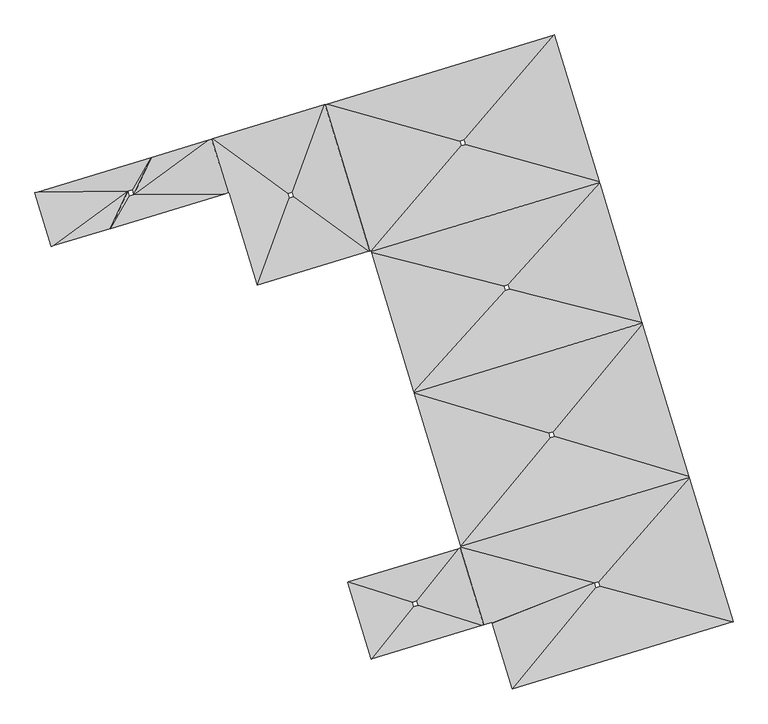
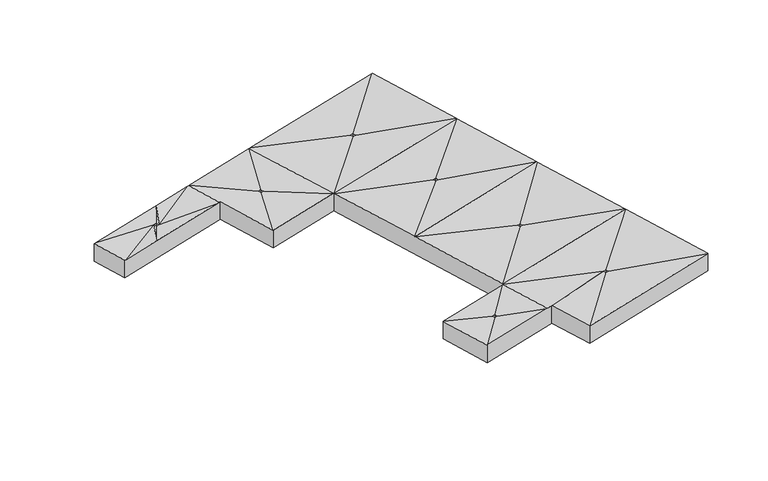
"""IFC4 building model written with IfcOpenShell, lengths in millimetres: proxy geometry, layer-410_topoId-1346273_creation_time-2021_Oct_27_15_18_18_ : layer-410_topoId-1346273_creation_time-2021_Oct_27_15_18_18_."""

from ifc_helpers import new_model, si_unit, origin, place, context, project, spatial, faceted_brep, source, transform, mapped, element, save


def generic_models_39dac30f(model_context):
    return source(origin(), model_context, "Body", "Brep", [
        faceted_brep([(28125.7662588, -17147.5862588, 474910.0155273), (10320.9487086, -22562.4314291, 474910.0155273), (8691.5481583, -17204.7223877, 474910.0155273), (-1028.2339046, -20160.7291608, 474910.0155273), (-2912.6258867, -13964.5670218, 474910.0155273), (6232.0389055, -11183.4693329, 474910.0155273), (-1053.4223403, 12772.2083054, 474910.0155273), (-10198.0872101, 9991.1094522, 474910.0155273), (-12471.5344882, 17466.5380451, 474910.0155273), (-26809.1523566, 13106.1448971, 474910.0155273), (-28125.7662527, 17435.3652172, 474910.0155273), (13736.4526166, 30166.6114523, 474910.0155273), (-20144.7843384, 17288.7016937, 474910.0155273), (-20261.1702576, 17671.3946136, 474910.0155273), (-20643.8631775, 17555.0086945, 474910.0155273), (-20527.4772583, 17172.3157745, 474910.0155273), (13370.0862305, -2328.9415649, 474910.0155273), (13752.7791504, -2212.5552097, 474910.0155273), (13636.3943939, -1829.8628712, 474910.0155273), (13253.7003113, -1946.247337, 474910.0155273), (10139.1450714, 9669.6086151, 474910.0155273), (10022.7579895, 10052.3026978, 474910.0155273), (9640.0656509, 9935.9167786, 474910.0155273), (9756.449826, 9553.2232773, 474910.0155273), (17312.0572449, -13915.987793, 474910.0155273), (16929.3631622, -14032.3713867, 474910.0155273), (17045.7490814, -14415.0654694, 474910.0155273), (17428.4420013, -14298.6795502, 474910.0155273), (2373.0752083, -15950.7356873, 474910.0155273), (2755.7692909, -15834.3486053, 474910.0155273), (2639.3830811, -15451.6545227, 474910.0155273), (2256.6897251, -15568.0416046, 474910.0155273), (6591.0546661, 21336.2557983, 474910.0155273), (6474.6681656, 21718.9487183, 474910.0155273), (6091.975827, 21602.5627991, 474910.0155273), (6208.3605835, 21219.8698792, 474910.0155273), (-7383.3045639, 17504.4268982, 474910.0155273), (-7765.9980652, 17388.040979, 474910.0155273), (-7649.612146, 17005.3468964, 474910.0155273), (-7266.9192261, 17121.7328156, 474910.0155273), (13736.4526166, 30166.6114523, 477196.9563735), (17337.0312354, 18327.3748578, 477196.9563736), (17355.6091377, 18266.2879591, 477200.0071289), (17373.1332797, 18208.6659809, 477196.9563739), (20786.012385, 6986.6132293, 477196.9563604), (20803.5365983, 6928.9910163, 477200.0071289), (20822.8041265, 6865.6365256, 477196.9563601), (24563.609524, -5434.6865183, 477196.956334), (24582.8772052, -5498.0415121, 477200.0071289), (24601.0541471, -5557.8099932, 477196.9563339), (28125.7662588, -17147.5862588, 477196.9563725), (10022.7579907, 10052.3026981, 476910.0154846), (10139.1450714, 9669.6086151, 476910.0155273), (9756.4498265, 9553.2232758, 476910.0154978), (2406.0771892, 1396.8605102, 477196.9570659), (2423.6012978, 1339.238641, 477200.0078163), (6591.0546661, 21336.2557983, 476910.0155273), (6208.3605834, 21219.8698796, 476910.0155364), (-1042.9065397, 12737.6241389, 477196.956431), (-1024.3258936, 12676.5348712, 477200.0073352), (-28125.7662527, 17435.3652172, 477197.264433), (-27898.7824792, 17504.3961093, 477190.7574194), (-18764.6808399, 20282.2827155, 477190.7574657), (-18748.8130647, 20287.1084643, 477192.2013141), (-14156.112444, 21683.8524513, 477192.2012927), (-13883.8217202, 21766.6622102, 477200.0071289), (-13811.6386368, 21788.6147162, 477196.711422), (-4811.3393377, 24525.8090088, 477196.7114045), (-4739.1558066, 24547.7616509, 477200.0071289), (-4589.3130727, 24593.3322105, 477195.2290651), (13682.2837137, 30150.1374655, 477195.2290779), (-20261.1702576, 17671.3946136, 476999.9821289), (-20144.7843384, 17288.7016937, 476999.9821289), (8020.7580555, -17408.7249131, 477200.0072194), (8691.5481608, -17204.722387, 477178.6175937), (8704.8017052, -17248.3019934, 477178.6175954), (16929.3631622, -14032.3713867, 476910.0155273), (6221.1191764, -11147.5636584, 477196.9562258), (6232.0389012, -11183.4693342, 477196.9562273), (6136.3656478, -11212.5657166, 477200.0069803), (2442.8686671, 1275.8846717, 477196.9562276), (13253.700312, -1946.2473395, 476910.0155846), (13636.3943939, -1829.8628712, 476910.0155273), (6474.6681656, 21718.9487183, 476910.0155273), (6202.9419645, -11087.794273, 477200.0067682), (17312.0572437, -13915.987789, 476910.0154428), (6183.6750397, -11024.4417655, 477196.9563724), (-1006.8017387, 12618.9128494, 477196.9563721), (-1053.4223403, 12772.2083054, 477196.956372), (9640.0656498, 9935.9167782, 476910.0154888), (13370.0862303, -2328.941565, 476910.015521), (13752.7791512, -2212.5552123, 476910.0154702), (28068.2902611, -17165.0660015, 477195.1236232), (10368.7396641, -22547.8971255, 477195.1236229), (10320.9487086, -22562.4314291, 477196.7504201), (17428.4420013, -14298.6795502, 476910.0155273), (17045.7490817, -14415.0654704, 476910.0155049), (7881.1577971, -17451.1805265, 477195.2267761), (-984.3046844, -20147.3692859, 477195.2266954), (-1028.2339046, -20160.7291608, 477196.7309708), (2755.7692909, -15834.3486053, 477049.9883789), (2373.0752065, -15950.7356815, 477049.9885037), (6091.9758266, 21602.5628004, 476910.0154974), (-12889.8650569, 17339.3142788, 477190.7574189), (-12567.2078521, 17437.4416161, 477200.0071289), (-2912.6258867, -13964.5670218, 477196.730971), (2256.6897251, -15568.0416046, 477049.9883789), (-2868.6966966, -13951.2070954, 477195.2267039), (-7383.3045648, 17504.4268979, 476999.9821493), (-7266.9192261, 17121.7328156, 476999.9821289), (-1221.2774175, 12721.1616295, 477196.7115505), (-1149.0957229, 12743.1118717, 477200.0071646), (-12471.5344882, 17466.5380451, 477195.6389198), (-22023.9665536, 14561.4278862, 477190.7574501), (-22039.8343554, 14556.6021296, 477192.201301), (-26632.5344618, 13159.8583846, 477192.2012731), (-26809.1523566, 13106.1448971, 477197.2644337), (-20527.4772591, 17172.3157772, 476999.982159), (8718.2324863, -17292.4643893, 477196.7504202), (-10198.0872101, 9991.1094522, 477196.7114132), (-7649.612146, 17005.3468964, 476999.9821289), (-10207.5573128, 10022.2441264, 477195.6387725), (-7765.9980652, 17388.040979, 476999.9821289), (5996.7629108, -11255.0220404, 477195.2266957), (2639.3830823, -15451.6545268, 477049.9884692), (-20643.8631775, 17555.0086945, 476999.9821289)], [[[0, 1, 2, 3, 4, 5, 6, 7, 8, 9, 10, 11], [12, 13, 14, 15], [16, 17, 18, 19], [20, 21, 22, 23], [24, 25, 26, 27], [28, 29, 30, 31], [32, 33, 34, 35], [36, 37, 38, 39]], [[0, 11, 40, 41, 42, 43, 44, 45, 46, 47, 48, 49, 50]], [[44, 43, 51, 52]], [[45, 44, 52, 53, 54, 55]], [[42, 41, 56, 57, 58, 59]], [[11, 10, 60, 61, 62, 63, 64, 65, 66, 67, 68, 69, 70, 40]], [[63, 62, 71, 72]], [[13, 12, 72, 71]], [[64, 63, 72]], [[73, 74, 75, 76, 77, 78, 79]], [[46, 45, 55, 80, 81, 82]], [[41, 40, 70, 83, 56]], [[49, 48, 84, 77, 76, 85]], [[6, 5, 78, 77, 84, 86, 80, 55, 54, 87, 59, 58, 88]], [[54, 53, 89, 87]], [[81, 80, 86, 90]], [[33, 32, 56, 83]], [[48, 47, 91, 90, 86, 84]], [[1, 0, 50, 92, 93, 94]], [[93, 92, 95, 96]], [[3, 2, 74, 73, 97, 98, 99]], [[98, 97, 100, 101]], [[70, 69, 102, 83]], [[65, 64, 72, 103, 104]], [[4, 3, 99, 105]], [[99, 98, 101, 106, 107, 105]], [[16, 19, 81, 90]], [[108, 109, 110, 111, 68, 67]], [[47, 46, 82, 91]], [[50, 49, 85, 95, 92]], [[23, 22, 89, 53]], [[29, 28, 101, 100]], [[19, 18, 82, 81]], [[43, 42, 59, 87, 89, 51]], [[36, 39, 109, 108]], [[58, 57, 102, 69, 68, 111, 88]], [[9, 8, 112, 104, 103, 113, 114, 115, 116]], [[103, 72, 117, 113]], [[34, 33, 83, 102]], [[2, 1, 94, 118, 75, 74]], [[94, 93, 96, 76, 118]], [[7, 6, 88, 111, 110, 119]], [[110, 109, 120, 121, 119]], [[39, 38, 120, 109]], [[8, 7, 119, 121, 112]], [[66, 65, 104, 112, 121, 120, 122]], [[5, 4, 105, 107, 123, 79, 78]], [[107, 106, 124, 123]], [[62, 61, 125, 71]], [[14, 13, 71, 125]], [[12, 15, 117, 72]], [[27, 26, 96, 95]], [[73, 79, 123, 124, 100, 97]], [[115, 114, 125]], [[10, 9, 116, 60]], [[61, 60, 116, 115, 125]], [[38, 37, 122, 120]], [[114, 113, 117, 125]], [[15, 14, 125, 117]], [[35, 34, 102, 57]], [[17, 16, 90, 91]], [[32, 35, 57, 56]], [[24, 27, 95, 85]], [[25, 24, 85, 76]], [[22, 21, 51, 89]], [[31, 30, 124, 106]], [[26, 25, 76, 96]], [[76, 75, 118]], [[28, 31, 106, 101]], [[30, 29, 100, 124]], [[21, 20, 52, 51]], [[20, 23, 53, 52]], [[67, 66, 122, 108]], [[18, 17, 91, 82]], [[37, 36, 108, 122]]]),
    ])


if __name__ == "__main__":
    model = new_model("IFC4")
    model_context = context("Model", 3, world=origin())
    ifc_project = project(units=[si_unit("LENGTHUNIT", "METRE", prefix="MILLI")], contexts=[model_context])
    site = spatial("IfcSite", under=ifc_project)
    building = spatial("IfcBuilding", under=site)
    placement = place(None, origin())
    generic_models_shape = generic_models_39dac30f(model_context)
    element("IfcBuildingElementProxy", 1, Name="layer-410_topoId-1346273_creation_time-2021_Oct_27_15_18_18_ : layer-410_topoId-1346273_creation_time-2021_Oct_27_15_18_18_", ObjectType="layer-410_topoId-1346273_creation_time-2021_Oct_27_15_18_18_ : layer-410_topoId-1346273_creation_time-2021_Oct_27_15_18_18_", at=placement, inside=building, context=model_context, shape_type="MappedRepresentation", body=[
        mapped(generic_models_shape, transform((0.0, 0.0, 0.0), x_axis=(1.0, 0.0, 0.0), y_axis=(0.0, 1.0, 0.0), z_axis=(0.0, 0.0, 1.0))),
    ])
    save(model, "model.ifc")

# Revit data of these elements
# Project information
#   Дата утверждения проекта = "Projekt Datum"
#   Статус проекта = "Projekt  Status"
#   Заказчик = "Bauherr"
#   Адрес проекта = "Projektadresse"
#   Наименование проекта = "Projektname"
#   Номер проекта = "01212"
#   Verfasser Firma 1 = "Firma"
#   Verfasser Firma 2 = "Firma"
#   Verfasser PLZ Ort = "PLZ Ort"
#   Verfasser Strasse = "Strasse"
#   Verfasser Telefon = "Telefon"
#   Verfasser Telefax = "Telefax"
#   Verfasser eMail = "eMail"
#   Extensions.Parameters = "2011.5"
#   Document GUID = "cf571a61-1359-4164-9d26-57dc57f15400"
# Type "layer-410_topoId-1346273_creation_time-2021_Oct_27_15_18_18_ : layer-410_topoId-1346273_creation_time-2021_Oct_27_15_18_18_"
#   Default Elevation = 0
# Element 1 (IfcBuildingElementProxy, "layer-410_topoId-1346273_creation_time-2021_Oct_27_15_18_18_ : layer-410_topoId-1346273_creation_time-2021_Oct_27_15_18_18_")
#   Materials on its faces: "Naturstein - Granit"
# Materials
#   "Naturstein - Granit": class "Stein", colour RGB 129 131 128, transparency 0, Cost = 0
